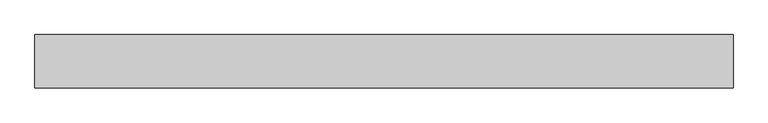
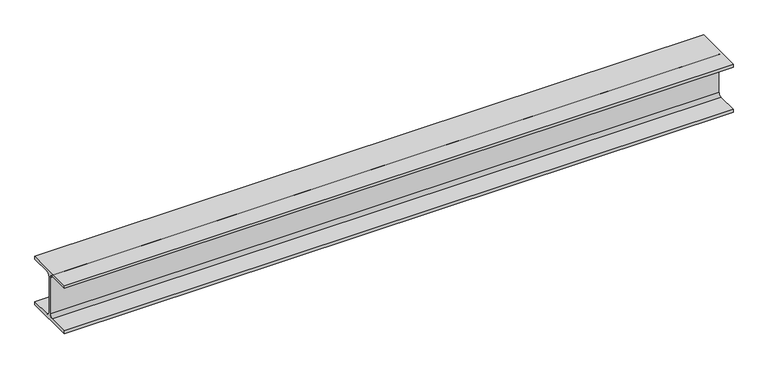
"""IFC4 building model written with IfcOpenShell, lengths in millimetres: beam geometry, 0912_Steel Framing_H-KSD3502 : H_SB_ASB_H-200x200x8x12."""

from ifc_helpers import new_model, si_unit, point, frame, frame_2d, origin, place, context, project, spatial, polyline, circle_curve, trimmed, segment, composite_curve, outline, extrude, source, transform, mapped, element, save


def beam_192a384f(model_context):
    return source(origin(), model_context, "Body", "SweptSolid", [
        extrude(outline(composite_curve([segment(polyline([(100.0, -88.0), (100.0, -100.0), (-100.0, -100.0), (-100.0, -88.0), (-17.0, -88.0)]), True, "CONTINUOUS"), segment(trimmed(circle_curve(frame_2d((-17.0, -75.0)), 13.0), [point((-17.0, -88.0))], [point((-4.0, -75.0))], True, "CARTESIAN"), True, "CONTINUOUS"), segment(polyline([(-4.0, -75.0), (-4.0, 75.0)]), True, "CONTINUOUS"), segment(trimmed(circle_curve(frame_2d((-17.0, 75.0)), 13.0), [point((-4.0, 75.0))], [point((-17.0, 88.0))], True, "CARTESIAN"), True, "CONTINUOUS"), segment(polyline([(-17.0, 88.0), (-100.0, 88.0), (-100.0, 100.0), (100.0, 100.0), (100.0, 88.0), (17.0, 88.0)]), True, "CONTINUOUS"), segment(trimmed(circle_curve(frame_2d((17.0, 75.0)), 13.0), [point((17.0, 88.0))], [point((4.0, 75.0))], True, "CARTESIAN"), True, "CONTINUOUS"), segment(polyline([(4.0, 75.0), (4.0, -75.0)]), True, "CONTINUOUS"), segment(trimmed(circle_curve(frame_2d((17.0, -75.0)), 13.0), [point((4.0, -75.0))], [point((17.0, -88.0))], True, "CARTESIAN"), True, "CONTINUOUS"), segment(polyline([(17.0, -88.0), (100.0, -88.0)]), True, "CONTINUOUS")], self_intersect=False)), frame((-1295.3889401, 0.0, 0.0), z_axis=(1.0, 0.0, 0.0), x_axis=(0.0, 1.0, 0.0)), (0.0, 0.0, 1.0), 2624.3471578),
    ])


if __name__ == "__main__":
    model = new_model("IFC4")
    model_context = context("Model", 3, world=origin())
    ifc_project = project(units=[si_unit("LENGTHUNIT", "METRE", prefix="MILLI")], contexts=[model_context])
    site = spatial("IfcSite", under=ifc_project)
    building = spatial("IfcBuilding", under=site)
    placement = place(None, origin())
    beam_shape = beam_192a384f(model_context)
    element("IfcBeam", 1, ObjectType="0912_Steel Framing_H-KSD3502 : H_SB_ASB_H-200x200x8x12", at=placement, inside=building, context=model_context, shape_type="MappedRepresentation", body=[
        mapped(beam_shape, transform((0.0, 0.0, 0.0), x_axis=(1.0, 0.0, 0.0), y_axis=(0.0, 1.0, 0.0), z_axis=(0.0, 0.0, 1.0))),
    ])
    save(model, "model.ifc")

# Revit data of these elements
# Type "0912_Steel Framing_H-KSD3502 : H_SB_ASB_H-200x200x8x12"
#   H_WM Code_1 = "S01AA002-00001 | Main Steel Structure Fabrication Work | Shelter/Building | Medium Steel - Standard (90KG/M>Weight≥30KG/M) | Material: (   )"
#   H_WM Code_2 = "S03AA028-00001 | Main Steel Structure Erection Work | Shelter/Building | Medium Steel (90KG/M>Weight≥30KG/M) | Material: (   )"
#   H_WM Code_3 = "S01AA010-00001 | Main Steel Structure Fabrication Work | Shelter/Building | Steel Painting/Coating | for Non-Fireproofed Steel Surface, Surface Preparation, Primer, Second & Final Coat | Material: (   )"
#   H_Q'ty Cal Type Tag = "SB-Q2"
#   Width = 20.0 cm
#   Web Thickness = 0.8 cm
#   Web Fillet = 1.3 cm
#   Warping Constant = 141000.0 cm⁶
#   W = 0
#   Torsional Moment of Inertia = 26.2485 cm⁴
#   Section Area = 63.53 cm²
#   Plastic Modulus weak axis = 244.0 cm³
#   Plastic Modulus strong axis = 525.0 cm³
#   Perimeter = 1.16 m²/m
#   Nominal Weight = 49.90 kgf/m
#   Moment of Inertia weak axis = 1600.00 cm⁴
#   Moment of Inertia strong axis = 4720.00 cm⁴
#   Height = 20.0 cm
#   Flange Thickness = 1.2 cm
#   Elastic Modulus weak axis = 160.0 cm³
#   Elastic Modulus strong axis = 472.0 cm³
#   Centroid Vertical = 10.0 cm
#   Centroid Horizontal = 10.0 cm
#   Ix = 47200000
#   Length [instance default] = 1.5240 m
#   Zx = 525000
#   b = 0.2000 m
#   h = 0.2000 m
#   r = 0.0130 m
#   s = 0.0080 m
#   t = 0.0120 m
#   A = 0.006353 m²
#   Structural Material [instance default] = Steel, 45-345
#   Assembly Code = ""
# Element 1 (IfcBeam, "0912_Steel Framing_H-KSD3502 : H_SB_ASB_H-200x200x8x12")
#   Structural Material = none
# Materials
#   "Steel, 45-345": class "Metal", colour RGB 189 187 185, transparency 0, Description = "Steel 345 MPa", Cost = 0
